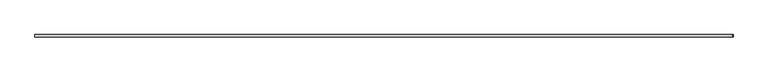
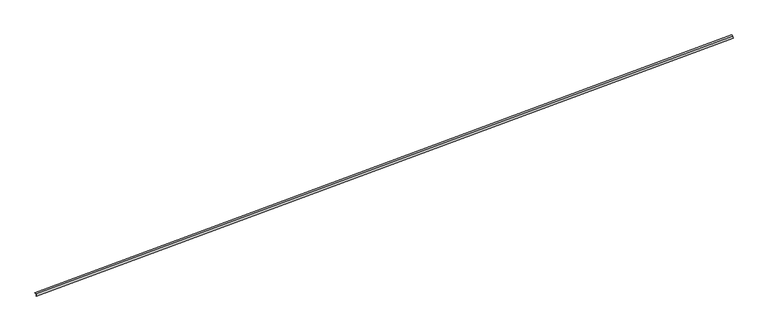
"""IFC4 building model written with IfcOpenShell, lengths in millimetres: proxy geometry, Generic Models 2:Generic Models 2:310765:Generic Models 2:310765 : Generic Models 2:Generic Models 2:310765:7 : Generic Models 2:Generic Models 2:310765:Generic Models 2:310765 : Generic Models 2:Generic Models 2:310765:300385."""

from ifc_helpers import new_model, si_unit, frame, origin, place, context, project, spatial, polyline, outline, extrude, source, transform, mapped, element, save


def generic_models_34207558(model_context):
    return source(origin(), model_context, "Body", "SweptSolid", [
        extrude(outline(polyline([(38.1, 0.0), (38.1, -50.8), (33.3375001, -50.8), (33.3375001, -4.7625), (-12.7, -4.7625), (-12.7, 0.0), (38.1, 0.0)])), frame((563237.7074879, -578778.4413841, 3754.5561022), z_axis=(0.9991330730923568, 0.0, 0.04163054471206785), x_axis=(-0.04163054471206785, 0.0, 0.9991330730923568)), (0.0, 0.0, 1.0), 15852.9020761),
    ])


if __name__ == "__main__":
    model = new_model("IFC4")
    model_context = context("Model", 3, world=origin())
    ifc_project = project(units=[si_unit("LENGTHUNIT", "METRE", prefix="MILLI")], contexts=[model_context])
    site = spatial("IfcSite", under=ifc_project)
    building = spatial("IfcBuilding", under=site)
    placement = place(None, origin())
    generic_models_shape = generic_models_34207558(model_context)
    element("IfcBuildingElementProxy", 1, Name="Generic Models 2:Generic Models 2:310765:Generic Models 2:310765 : Generic Models 2:Generic Models 2:310765:7 : Generic Models 2:Generic Models 2:310765:Generic Models 2:310765 : Generic Models 2:Generic Models 2:310765:300385", ObjectType="Generic Models 2:Generic Models 2:310765:Generic Models 2:310765 : Generic Models 2:Generic Models 2:310765:7 : Generic Models 2:Generic Models 2:310765:Generic Models 2:310765 : Generic Models 2:Generic Models 2:310765:300385", at=placement, inside=building, context=model_context, shape_type="MappedRepresentation", body=[
        mapped(generic_models_shape, transform((0.0, 0.0, 0.0), x_axis=(1.0, 0.0, 0.0), y_axis=(0.0, 1.0, 0.0), z_axis=(0.0, 0.0, 1.0))),
    ])
    save(model, "model.ifc")

# Revit data of these elements
# Type "Generic Models 2:Generic Models 2:310765:Generic Models 2:310765 : Generic Models 2:Generic Models 2:310765:7 : Generic Models 2:Generic Models 2:310765:Generic Models 2:310765 : Generic Models 2:Generic Models 2:310765:300385"
#   NameOverride = "Generic Models 2:Generic Models 2:310765:Generic Models 2:310765 : Generic Models 2:Generic Models 2:310765:300385"
#   ObjectTypeOverride = "Generic Models 2:310765 : Generic Models 2:Generic Models 2:310765"
#   Reference = "Generic Models 2"
#   Tag = "300385"
# Element 1 (IfcBuildingElementProxy, "Generic Models 2:Generic Models 2:310765:Generic Models 2:310765 : Generic Models 2:Generic Models 2:310765:7 : Generic Models 2:Generic Models 2:310765:Generic Models 2:310765 : Generic Models 2:Generic Models 2:310765:300385")
#   Materials on its faces: "2 X 2 X 3/16 GAL. STEEL ANGLE TO FASTEN INTERIOR PLYWOOD."
# Materials
#   "2 X 2 X 3/16 GAL. STEEL ANGLE TO FASTEN INTERIOR PLYWOOD.": class "Unassigned", colour RGB 210 209 208, transparency 0, Keynote = "M05121300.02", Cost = 0
